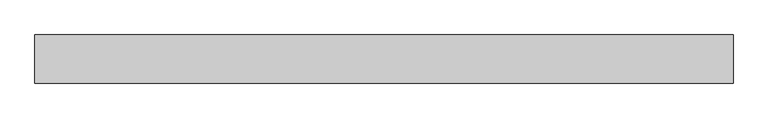
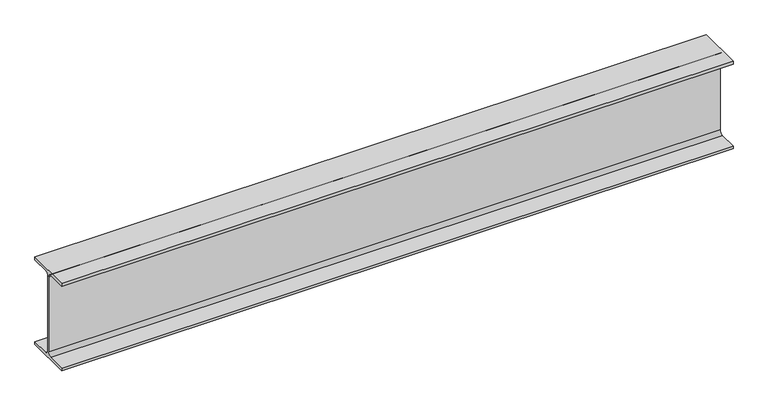
"""IFC4 building model written with IfcOpenShell, lengths in millimetres: beam geometry, 0912_Steel Framing_H-KSD3502 : H_SB_ASB_H-350x175x7x11."""

from ifc_helpers import new_model, si_unit, point, frame, frame_2d, origin, place, context, project, spatial, polyline, circle_curve, trimmed, segment, composite_curve, outline, extrude, source, transform, mapped, element, save


def beam_15665a20(model_context):
    return source(origin(), model_context, "Body", "SweptSolid", [
        extrude(outline(composite_curve([segment(polyline([(87.5, -164.0), (87.5, -175.0), (-87.5, -175.0), (-87.5, -164.0), (-17.5, -164.0)]), True, "CONTINUOUS"), segment(trimmed(circle_curve(frame_2d((-17.5, -150.0)), 14.0), [point((-17.5, -164.0))], [point((-3.5, -150.0))], True, "CARTESIAN"), True, "CONTINUOUS"), segment(polyline([(-3.5, -150.0), (-3.5, 150.0)]), True, "CONTINUOUS"), segment(trimmed(circle_curve(frame_2d((-17.5, 150.0)), 14.0), [point((-3.5, 150.0))], [point((-17.5, 164.0))], True, "CARTESIAN"), True, "CONTINUOUS"), segment(polyline([(-17.5, 164.0), (-87.5, 164.0), (-87.5, 175.0), (87.5, 175.0), (87.5, 164.0), (17.5, 164.0)]), True, "CONTINUOUS"), segment(trimmed(circle_curve(frame_2d((17.5, 150.0)), 14.0), [point((17.5, 164.0))], [point((3.5, 150.0))], True, "CARTESIAN"), True, "CONTINUOUS"), segment(polyline([(3.5, 150.0), (3.5, -150.0)]), True, "CONTINUOUS"), segment(trimmed(circle_curve(frame_2d((17.5, -150.0)), 14.0), [point((3.5, -150.0))], [point((17.5, -164.0))], True, "CARTESIAN"), True, "CONTINUOUS"), segment(polyline([(17.5, -164.0), (87.5, -164.0)]), True, "CONTINUOUS")], self_intersect=False)), frame((-1244.2450896, 0.0, 0.0), z_axis=(1.0, 0.0, 0.0), x_axis=(0.0, 1.0, 0.0)), (0.0, 0.0, 1.0), 2540.0189947),
    ])


if __name__ == "__main__":
    model = new_model("IFC4")
    model_context = context("Model", 3, world=origin())
    ifc_project = project(units=[si_unit("LENGTHUNIT", "METRE", prefix="MILLI")], contexts=[model_context])
    site = spatial("IfcSite", under=ifc_project)
    building = spatial("IfcBuilding", under=site)
    placement = place(None, origin())
    beam_shape = beam_15665a20(model_context)
    element("IfcBeam", 1, ObjectType="0912_Steel Framing_H-KSD3502 : H_SB_ASB_H-350x175x7x11", at=placement, inside=building, context=model_context, shape_type="MappedRepresentation", body=[
        mapped(beam_shape, transform((0.0, 0.0, 0.0), x_axis=(1.0, 0.0, 0.0), y_axis=(0.0, 1.0, 0.0), z_axis=(0.0, 0.0, 1.0))),
    ])
    save(model, "model.ifc")

# Revit data of these elements
# Type "0912_Steel Framing_H-KSD3502 : H_SB_ASB_H-350x175x7x11"
#   H_WM Code_1 = "S01AA002-00001 | Main Steel Structure Fabrication Work | Shelter/Building | Medium Steel - Standard (90KG/M>Weight≥30KG/M) | Material: (   )"
#   H_WM Code_2 = "S03AA028-00001 | Main Steel Structure Erection Work | Shelter/Building | Medium Steel (90KG/M>Weight≥30KG/M) | Material: (   )"
#   H_WM Code_3 = "S01AA010-00001 | Main Steel Structure Fabrication Work | Shelter/Building | Steel Painting/Coating | for Non-Fireproofed Steel Surface, Surface Preparation, Primer, Second & Final Coat | Material: (   )"
#   H_Q'ty Cal Type Tag = "SB-Q2"
#   Width = 17.5 cm
#   Web Thickness = 0.7 cm
#   Web Fillet = 1.4 cm
#   Warping Constant = 282000.0 cm⁶
#   W = 0
#   Torsional Moment of Inertia = 19.4042 cm⁴
#   Section Area = 63.14 cm²
#   Plastic Modulus weak axis = 174.0 cm³
#   Plastic Modulus strong axis = 868.0 cm³
#   Perimeter = 1.36 m²/m
#   Nominal Weight = 49.60 kgf/m
#   Moment of Inertia weak axis = 984.00 cm⁴
#   Moment of Inertia strong axis = 13600.00 cm⁴
#   Height = 35.0 cm
#   Flange Thickness = 1.1 cm
#   Elastic Modulus weak axis = 112.0 cm³
#   Elastic Modulus strong axis = 775.0 cm³
#   Centroid Vertical = 17.5 cm
#   Centroid Horizontal = 8.75 cm
#   Ix = 136000000
#   Length [instance default] = 1.5240 m
#   Zx = 868000
#   b = 0.1750 m
#   h = 0.3500 m
#   r = 0.0140 m
#   s = 0.0070 m
#   t = 0.0110 m
#   A = 0.006314 m²
#   Structural Material [instance default] = Steel, 45-345
#   Assembly Code = ""
# Element 1 (IfcBeam, "0912_Steel Framing_H-KSD3502 : H_SB_ASB_H-350x175x7x11")
#   Structural Material = none
# Materials
#   "Steel, 45-345": class "Metal", colour RGB 189 187 185, transparency 0, Description = "Steel 345 MPa", Cost = 0
